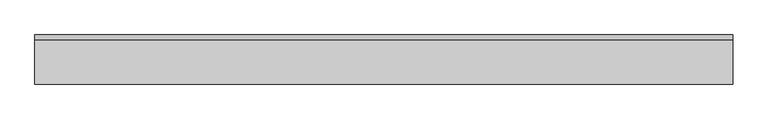
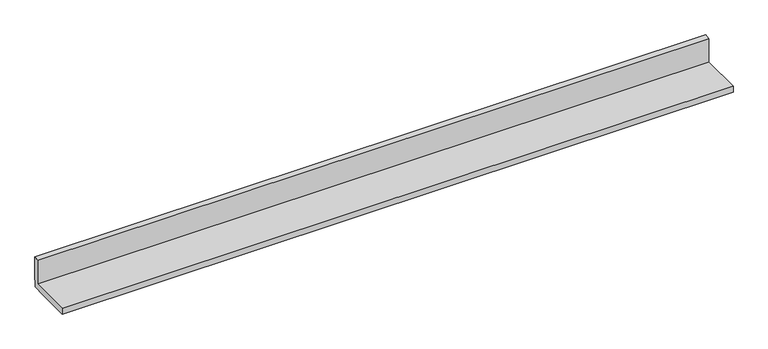
"""IFC4 building model written with IfcOpenShell, lengths in millimetres: proxy geometry, Gypsum017 33610 : Gypsum017 33610."""

import ifcopenshell
import ifcopenshell.guid

model = None  # the IFC model being written
_history = None  # IfcOwnerHistory: only IFC2X3 demands one
_inside = {}  # id of a spatial element -> (the spatial element, [elements in it])
_under = {}  # id of a project, library or spatial element -> (it, [spatial elements below it])
_declared = {}  # id of a project -> (the project, [libraries it declares])
_typed = {}  # id of a type object -> (the type object, [elements of that type])
_made_of = {}  # id of a material, layer set ... -> (it, [elements and type objects made of it])


def new_model(schema):
    """Start an empty IFC model of exactly this schema.

    Asked for "IFC4X3", IfcOpenShell would pick the latest addendum, in which some entities
    have other attributes; the version numbers below select the first issue.
    IFC2X3 requires an IfcOwnerHistory on every rooted entity: one is made here for all.
    """
    global model, _history
    if schema == "IFC4X3":
        model = ifcopenshell.file(schema_version=(4, 3, 0, 0))
    else:
        model = ifcopenshell.file(schema=schema)
    _inside.clear()
    _under.clear()
    _declared.clear()
    _typed.clear()
    _made_of.clear()
    _history = None
    if model.schema == "IFC2X3":
        org = make("IfcOrganization", Name="unknown")
        user = make(
            "IfcPersonAndOrganization",
            ThePerson=make("IfcPerson", FamilyName="unknown"),
            TheOrganization=org,
        )
        app = make(
            "IfcApplication",
            ApplicationDeveloper=org,
            Version="unknown",
            ApplicationFullName="unknown",
            ApplicationIdentifier="unknown",
        )
        _history = make(
            "IfcOwnerHistory",
            OwningUser=user,
            OwningApplication=app,
            ChangeAction="ADDED",
            CreationDate=0,
        )
    return model


def make(cls, **values):
    """One entity of the class cls with the attributes given. An attribute that is None is left unset."""
    return model.create_entity(
        cls, **{name: value for name, value in values.items() if value is not None}
    )


def rooted(cls, **values):
    """An entity with a GlobalId (a new one), such as an element, a storey or a relation."""
    return make(cls, GlobalId=ifcopenshell.guid.new(), OwnerHistory=_history, **values)


def si_unit(unit_type, name, prefix=None):
    """IfcSIUnit, for example si_unit("LENGTHUNIT", "METRE", prefix="MILLI")."""
    return make("IfcSIUnit", UnitType=unit_type, Prefix=prefix, Name=name)


def assignment(units):
    """IfcUnitAssignment: the units of a project."""
    return None if units is None else make("IfcUnitAssignment", Units=units)


def point(xyz):
    """IfcCartesianPoint."""
    return None if xyz is None else make("IfcCartesianPoint", Coordinates=xyz)


def direction(xyz):
    """IfcDirection."""
    return None if xyz is None else make("IfcDirection", DirectionRatios=xyz)


def frame(location, z_axis=None, x_axis=None):
    """IfcAxis2Placement3D, a coordinate frame: its origin and axes. An axis left out is left unset."""
    return make(
        "IfcAxis2Placement3D",
        Location=point(location),
        Axis=direction(z_axis),
        RefDirection=direction(x_axis),
    )


def origin():
    """The frame at (0, 0, 0) with its axes left unset."""
    return frame((0.0, 0.0, 0.0))


def place(relative_to, where):
    """IfcLocalPlacement: puts the frame where relative to a parent placement (None: the world)."""
    return make(
        "IfcLocalPlacement", PlacementRelTo=relative_to, RelativePlacement=where
    )


def context(
    kind, dimensions, precision=None, world=None, true_north=None, identifier=None
):
    """IfcGeometricRepresentationContext, for example the 3D "Model" context."""
    return make(
        "IfcGeometricRepresentationContext",
        ContextIdentifier=identifier,
        ContextType=kind,
        CoordinateSpaceDimension=dimensions,
        Precision=precision,
        WorldCoordinateSystem=world,
        TrueNorth=true_north,
    )


def project(units=None, contexts=None):
    """IfcProject with its units and contexts."""
    return rooted(
        "IfcProject",
        Name="project",
        RepresentationContexts=contexts,
        UnitsInContext=assignment(units),
    )


def spatial(cls, under=None, at=None, **own):
    """A site, building, storey or space (cls), placed at a placement, below another one or the project."""
    s = rooted(cls, ObjectPlacement=at, **own)
    if under is not None:
        _under.setdefault(under.id(), (under, []))[1].append(s)
    return s


def polyline(points):
    """IfcPolyline through the points."""
    return make("IfcPolyline", Points=[point(p) for p in points])


def outline(outer, holes=None, kind="AREA"):
    """IfcArbitraryClosedProfileDef: a profile drawn as a closed curve; with holes, ...WithVoids."""
    if holes is None:
        return make("IfcArbitraryClosedProfileDef", ProfileType=kind, OuterCurve=outer)
    return make(
        "IfcArbitraryProfileDefWithVoids",
        ProfileType=kind,
        OuterCurve=outer,
        InnerCurves=holes,
    )


def extrude(swept, where, along, depth):
    """IfcExtrudedAreaSolid: the profile swept, set in the frame where, extruded along a direction by depth."""
    return make(
        "IfcExtrudedAreaSolid",
        SweptArea=swept,
        Position=where,
        ExtrudedDirection=direction(along),
        Depth=depth,
    )


def shape(context_of_items, identifier, shape_type, items):
    """IfcShapeRepresentation: the items that make up one representation, for example the "Body"."""
    return make(
        "IfcShapeRepresentation",
        ContextOfItems=context_of_items,
        RepresentationIdentifier=identifier,
        RepresentationType=shape_type,
        Items=items,
    )


def source(mapping_origin, context_of_items, identifier, shape_type, items):
    """IfcRepresentationMap: a shape defined once, which mapped items show again and again."""
    return make(
        "IfcRepresentationMap",
        MappingOrigin=mapping_origin,
        MappedRepresentation=shape(context_of_items, identifier, shape_type, items),
    )


def transform(
    local_origin,
    x_axis=None,
    y_axis=None,
    z_axis=None,
    scale=None,
    scale2=None,
    scale3=None,
    uniform=True,
):
    """IfcCartesianTransformationOperator3D, or its non-uniform kind. x_axis, y_axis, z_axis: its Axis1, 2, 3."""
    if uniform:
        return make(
            "IfcCartesianTransformationOperator3D",
            Axis1=direction(x_axis),
            Axis2=direction(y_axis),
            LocalOrigin=point(local_origin),
            Scale=scale,
            Axis3=direction(z_axis),
        )
    return make(
        "IfcCartesianTransformationOperator3DnonUniform",
        Axis1=direction(x_axis),
        Axis2=direction(y_axis),
        LocalOrigin=point(local_origin),
        Scale=scale,
        Axis3=direction(z_axis),
        Scale2=scale2,
        Scale3=scale3,
    )


def mapped(mapping_source, mapping_target):
    """IfcMappedItem: shows the shape of a source again, moved by a transform."""
    return make(
        "IfcMappedItem", MappingSource=mapping_source, MappingTarget=mapping_target
    )


def made_of(thing, what):
    """Note that an element or type object is made of a material, layer set ...; save() writes the relation."""
    if what is not None:
        _made_of.setdefault(what.id(), (what, []))[1].append(thing)
    return thing


def element(
    cls,
    number,
    at=None,
    inside=None,
    cuts=None,
    type_object=None,
    material=None,
    context=None,
    identifier="Body",
    shape_type=None,
    held_by="IfcProductDefinitionShape",
    body=None,
    shapes=None,
    **own,
):
    """One element of the class cls, such as IfcWall. Its Tag is "e" and its number.

    at: its placement. inside: the storey or other place that contains it. cuts: it is an
    opening in that element (IfcRelVoidsElement). A single representation is given by context,
    identifier, shape_type and body (its items); several are given by shapes. held_by: the class
    of the entity that holds the representations. save() writes the other relations.
    """
    e = rooted(cls, Tag="e%d" % number, ObjectPlacement=at, **own)
    if body is not None:
        shapes = [shape(context, identifier, shape_type, body)]
    if shapes is not None:
        e.Representation = make(held_by, Representations=shapes)
    if inside is not None:
        _inside.setdefault(inside.id(), (inside, []))[1].append(e)
    if cuts is not None:
        rooted(
            "IfcRelVoidsElement", RelatingBuildingElement=cuts, RelatedOpeningElement=e
        )
    if type_object is not None:
        _typed.setdefault(type_object.id(), (type_object, []))[1].append(e)
    return made_of(e, material)


def aggregate(whole, parts):
    """IfcRelAggregates: a whole, such as a stair, and the parts it consists of."""
    return rooted("IfcRelAggregates", RelatingObject=whole, RelatedObjects=parts)


def save(model, path):
    """Write the relations noted so far, then the file.

    IfcRelAggregates (storeys below a building ...), IfcRelContainedInSpatialStructure (elements
    in a storey), IfcRelDefinesByType, IfcRelAssociatesMaterial and IfcRelDeclares: one each for
    every whole, place, type object, material and project.
    """
    for whole, parts in _under.values():
        aggregate(whole, parts)
    for where, things in _inside.values():
        rooted(
            "IfcRelContainedInSpatialStructure",
            RelatedElements=things,
            RelatingStructure=where,
        )
    for kind, things in _typed.values():
        rooted("IfcRelDefinesByType", RelatedObjects=things, RelatingType=kind)
    for what, things in _made_of.values():
        rooted("IfcRelAssociatesMaterial", RelatedObjects=things, RelatingMaterial=what)
    for by, libraries in _declared.values():
        rooted("IfcRelDeclares", RelatingContext=by, RelatedDefinitions=libraries)
    model.write(path)


def generic_models_1a790526(model_context):
    return source(origin(), model_context, "Body", "SweptSolid", [
        extrude(outline(polyline([(-4376.7836914, 42583.1921875), (-4376.7836914, 42601.896), (-4250.2279008, 42601.896), (-4250.2279008, 42675.5351562), (-4235.9495263, 42678.9921875), (-4235.9495263, 42605.6253714), (-4237.2648904, 42605.6253714), (-4237.2648904, 42584.4721875), (-4258.4180743, 42584.4721875), (-4258.4180743, 42583.1921875), (-4376.7836914, 42583.1921875)])), frame((12383.0178845, 0.0, 0.0), z_axis=(1.0, 0.0, 0.0), x_axis=(0.0, 1.0, 0.0)), (0.0, 0.0, 1.0), 2000.0),
    ])


if __name__ == "__main__":
    model = new_model("IFC4")
    model_context = context("Model", 3, world=origin())
    ifc_project = project(units=[si_unit("LENGTHUNIT", "METRE", prefix="MILLI")], contexts=[model_context])
    site = spatial("IfcSite", under=ifc_project)
    building = spatial("IfcBuilding", under=site)
    placement = place(None, origin())
    generic_models_shape = generic_models_1a790526(model_context)
    element("IfcBuildingElementProxy", 1, Name="Gypsum017 33610 : Gypsum017 33610", ObjectType="Gypsum017 33610 : Gypsum017 33610", at=placement, inside=building, context=model_context, shape_type="MappedRepresentation", body=[
        mapped(generic_models_shape, transform((0.0, 0.0, 0.0), x_axis=(1.0, 0.0, 0.0), y_axis=(0.0, 1.0, 0.0), z_axis=(0.0, 0.0, 1.0))),
    ])
    save(model, "model.ifc")

# Revit data of these elements
# Type "Gypsum017 33610 : Gypsum017 33610"
#   NameOverride = "Gypsum017"
# Element 1 (IfcBuildingElementProxy, "Gypsum017 33610 : Gypsum017 33610")
#   Materials on its faces: "5/8\"  GYPSUM BOARD"
# Materials
#   "5/8\"  GYPSUM BOARD": class "Unassigned", colour RGB 255 255 255, transparency 0, Cost = 0
